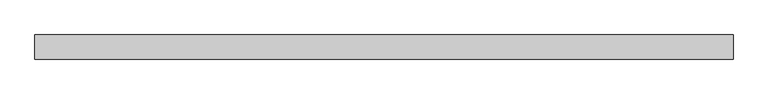
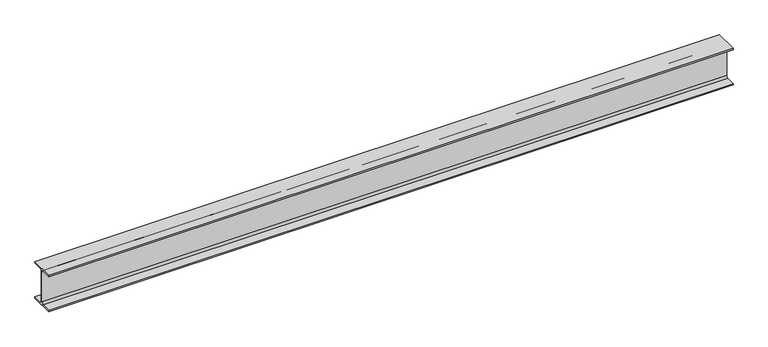
"""IFC4 building model written with IfcOpenShell, lengths in millimetres: beam geometry, 0912_Steel Framing_H-KSD3502 : H_SB_ASB_H-488x300x11x18."""

from ifc_helpers import new_model, si_unit, point, frame, frame_2d, origin, place, context, project, spatial, polyline, circle_curve, trimmed, segment, composite_curve, outline, extrude, source, transform, mapped, element, save


def beam_d635469f(model_context):
    return source(origin(), model_context, "Body", "SweptSolid", [
        extrude(outline(composite_curve([segment(polyline([(150.0, -226.0), (150.0, -244.0), (-150.0, -244.0), (-150.0, -226.0), (-31.5, -226.0)]), True, "CONTINUOUS"), segment(trimmed(circle_curve(frame_2d((-31.5, -200.0)), 26.0), [point((-31.5, -226.0))], [point((-5.5, -200.0))], True, "CARTESIAN"), True, "CONTINUOUS"), segment(polyline([(-5.5, -200.0), (-5.5, 200.0)]), True, "CONTINUOUS"), segment(trimmed(circle_curve(frame_2d((-31.5, 200.0)), 26.0), [point((-5.5, 200.0))], [point((-31.5, 226.0))], True, "CARTESIAN"), True, "CONTINUOUS"), segment(polyline([(-31.5, 226.0), (-150.0, 226.0), (-150.0, 244.0), (150.0, 244.0), (150.0, 226.0), (31.5, 226.0)]), True, "CONTINUOUS"), segment(trimmed(circle_curve(frame_2d((31.5, 200.0)), 26.0), [point((31.5, 226.0))], [point((5.5, 200.0))], True, "CARTESIAN"), True, "CONTINUOUS"), segment(polyline([(5.5, 200.0), (5.5, -200.0)]), True, "CONTINUOUS"), segment(trimmed(circle_curve(frame_2d((31.5, -200.0)), 26.0), [point((5.5, -200.0))], [point((31.5, -226.0))], True, "CARTESIAN"), True, "CONTINUOUS"), segment(polyline([(31.5, -226.0), (150.0, -226.0)]), True, "CONTINUOUS")], self_intersect=False)), frame((-4337.3, 0.0, 0.0), z_axis=(1.0, 0.0, 0.0), x_axis=(0.0, 1.0, 0.0)), (0.0, 0.0, 1.0), 8674.6),
    ])


if __name__ == "__main__":
    model = new_model("IFC4")
    model_context = context("Model", 3, world=origin())
    ifc_project = project(units=[si_unit("LENGTHUNIT", "METRE", prefix="MILLI")], contexts=[model_context])
    site = spatial("IfcSite", under=ifc_project)
    building = spatial("IfcBuilding", under=site)
    placement = place(None, origin())
    beam_shape = beam_d635469f(model_context)
    element("IfcBeam", 1, ObjectType="0912_Steel Framing_H-KSD3502 : H_SB_ASB_H-488x300x11x18", at=placement, inside=building, context=model_context, shape_type="MappedRepresentation", body=[
        mapped(beam_shape, transform((0.0, 0.0, 0.0), x_axis=(1.0, 0.0, 0.0), y_axis=(0.0, 1.0, 0.0), z_axis=(0.0, 0.0, 1.0))),
    ])
    save(model, "model.ifc")

# Revit data of these elements
# Type "0912_Steel Framing_H-KSD3502 : H_SB_ASB_H-488x300x11x18"
#   H_WM Code_1 = "S01AA001-00001 | Main Steel Structure Fabrication Work | Shelter/Building | Heavy Steel - Standard (Weight≥90KG/M) | Material: (   )"
#   H_WM Code_2 = "S03AA027-00001 | Main Steel Structure Erection Work | Shelter/Building | Heavy Steel (Weight≥90KG/M) | Material: (   )"
#   H_WM Code_3 = "S01AA010-00001 | Main Steel Structure Fabrication Work | Shelter/Building | Steel Painting/Coating | for Non-Fireproofed Steel Surface, Surface Preparation, Primer, Second & Final Coat | Material: (   )"
#   H_Q'ty Cal Type Tag = "SB-Q2"
#   Width = 30.0 cm
#   Web Thickness = 1.1 cm
#   Web Fillet = 2.6 cm
#   Warping Constant = 4470000.0 cm⁶
#   W = 0
#   Torsional Moment of Inertia = 137.492 cm⁴
#   Section Area = 163.5 cm²
#   Plastic Modulus weak axis = 830.0 cm³
#   Plastic Modulus strong axis = 3230.0 cm³
#   Perimeter = 2.11 m²/m
#   Nominal Weight = 128.00 kgf/m
#   Moment of Inertia weak axis = 8110.00 cm⁴
#   Moment of Inertia strong axis = 71000.00 cm⁴
#   Height = 48.8 cm
#   Flange Thickness = 1.8 cm
#   Elastic Modulus weak axis = 541.0 cm³
#   Elastic Modulus strong axis = 2910.0 cm³
#   Centroid Vertical = 24.4 cm
#   Centroid Horizontal = 15.0 cm
#   Ix = 710000000
#   Length [instance default] = 1.5240 m
#   Zx = 3230000
#   b = 0.3000 m
#   h = 0.4880 m
#   r = 0.0260 m
#   s = 0.0110 m
#   t = 0.0180 m
#   A = 0.01635 m²
#   Structural Material [instance default] = Steel, 45-345
#   Assembly Code = ""
# Element 1 (IfcBeam, "0912_Steel Framing_H-KSD3502 : H_SB_ASB_H-488x300x11x18")
#   Structural Material = none
# Materials
#   "Steel, 45-345": class "Metal", colour RGB 189 187 185, transparency 0, Description = "Steel 345 MPa", Cost = 0
